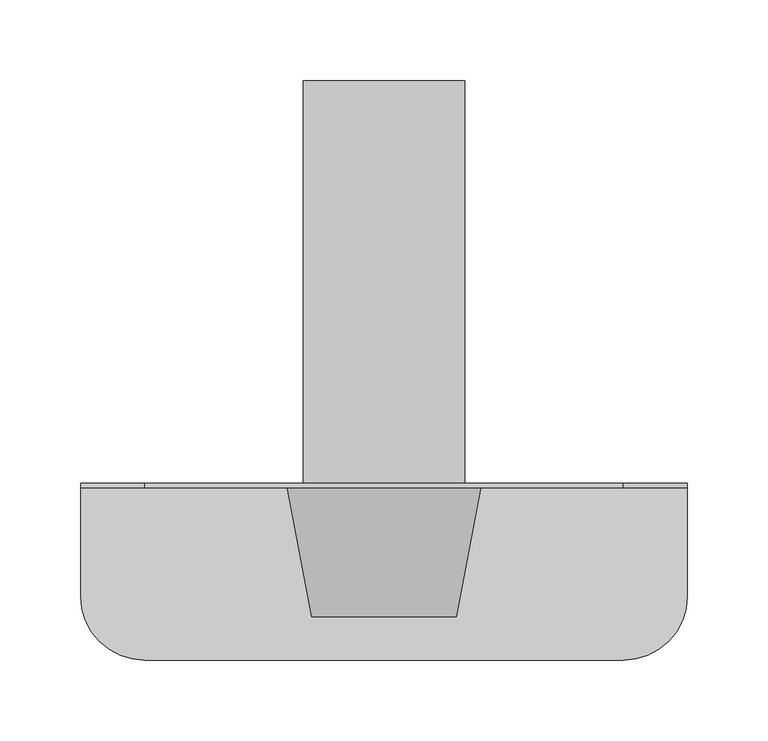
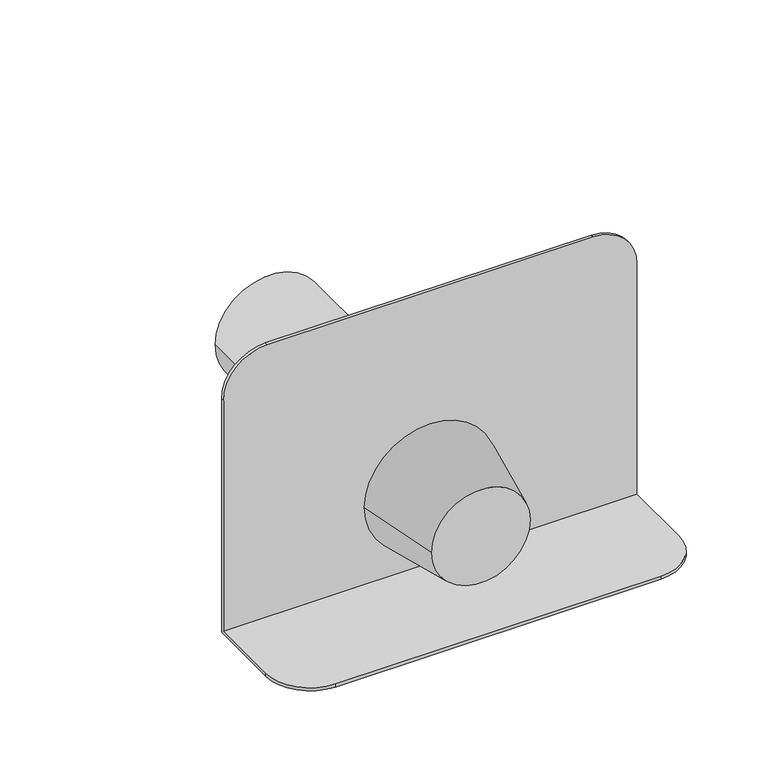
"""IFC4 building model written with IfcOpenShell, lengths in millimetres: proxy geometry, TN_Воронка парапетная ТехноНИКОЛЬ круглая_Тип 1 : Воронка ULTRA парапетная 110 ТехноНИКОЛЬ."""

from ifc_helpers import new_model, si_unit, frame, origin, place, context, project, spatial, polyline, circle_curve, source, transform, mapped, element, save
from ifc_brep_helpers import plane_surface, cylinder_surface, revolved_surface, advanced_brep


def specialty_equipment_830a0a6e(model_context):
    return source(origin(), model_context, "Body", "AdvancedBrep", [
        advanced_brep(
        [(-45.0, -83.0, 77.0), (45.0, -83.0, 77.0), (-60.0, -3.0, 77.0), (60.0, -3.0, 77.0)],
        [
            (0, 1, circle_curve(frame((0.0, -83.0, 77.0), z_axis=(0.0, -1.0, 0.0), x_axis=(-1.0, 0.0, 0.0)), 45.0)),
            (1, 0, circle_curve(frame((0.0, -83.0, 77.0), z_axis=(0.0, -1.0, 0.0), x_axis=(1.0, 0.0, 0.0)), 45.0)),
            (2, 3, circle_curve(frame((0.0, -3.0, 77.0), z_axis=(0.0, 1.0, 0.0), x_axis=(1.0, 0.0, 0.0)), 60.0)),
            (3, 2, circle_curve(frame((0.0, -3.0, 77.0), z_axis=(0.0, 1.0, 0.0), x_axis=(-1.0, 0.0, 0.0)), 60.0)),
            (3, 1),
            (0, 2),
        ],
        [
            plane_surface(frame((0.0, -83.0, 77.0), z_axis=(0.0, -1.0, 0.0), x_axis=(0.0, 0.0, -1.0))),
            plane_surface(frame((0.0, -3.0, 77.0), z_axis=(0.0, 1.0, 0.0), x_axis=(0.0, 0.0, -1.0))),
            revolved_surface(polyline([(-45.0, -83.0, 77.0), (-60.0, -3.0, 77.0)]), (0.0, -323.0, 77.0), (0.0, 1.0, 0.0)),
            revolved_surface(polyline([(45.0, -83.0, 77.0), (60.0, -3.0, 77.0)]), (0.0, -323.0, 77.0), (0.0, 1.0, 0.0)),
        ],
        [
            (0, [[1, 2]]),
            (1, [[3, 4]]),
            (2, [[-4, 5, -1, 6]]),
            (3, [[-3, -6, -2, -5]]),
        ],
    ),
        advanced_brep(
        [(-188.5, -70.0, 3.0), (-148.5, -110.0, 3.0), (148.5, -110.0, 3.0), (188.5, -70.0, 3.0), (188.5, -3.0, 3.0), (-188.5, -3.0, 3.0), (-188.5, 0.0, 0.0), (188.5, 0.0, 0.0), (188.5, -70.0, 0.0), (148.5, -110.0, 0.0), (-148.5, -110.0, 0.0), (-188.5, -70.0, 0.0), (188.5, 0.0, 225.0), (188.5, -3.0, 225.0), (-188.5, 0.0, 225.0), (-148.5, 0.0, 265.0), (148.5, 0.0, 265.0), (-50.0, 0.0, 77.0), (50.0, 0.0, 77.0), (-188.5, -3.0, 225.0), (148.5, -3.0, 265.0), (-148.5, -3.0, 265.0), (-47.0, -3.0, 77.0), (47.0, -3.0, 77.0), (-47.0, 0.0, 77.0), (47.0, 0.0, 77.0), (-50.0, 250.0, 77.0), (50.0, 250.0, 77.0), (-47.0, 250.0, 77.0), (47.0, 250.0, 77.0)],
        [
            (0, 1, circle_curve(frame((-148.5, -70.0, 3.0), z_axis=(0.0, 0.0, 1.0), x_axis=(1.0, 0.0, 0.0)), 40.0)),
            (1, 2),
            (2, 3, circle_curve(frame((148.5, -70.0, 3.0), z_axis=(0.0, 0.0, 1.0), x_axis=(1.0, 0.0, 0.0)), 40.0)),
            (3, 4),
            (4, 5),
            (5, 0),
            (6, 7),
            (7, 8),
            (8, 9, circle_curve(frame((148.5, -70.0, 0.0), z_axis=(0.0, 0.0, -1.0), x_axis=(1.0, 0.0, 0.0)), 40.0)),
            (9, 10),
            (10, 11, circle_curve(frame((-148.5, -70.0, 0.0), z_axis=(0.0, 0.0, -1.0), x_axis=(1.0, 0.0, 0.0)), 40.0)),
            (11, 6),
            (0, 11),
            (10, 1),
            (9, 2),
            (8, 3),
            (7, 12),
            (12, 13),
            (13, 4),
            (6, 14),
            (14, 15, circle_curve(frame((-148.5, 0.0, 225.0), z_axis=(0.0, 1.0, 0.0), x_axis=(1.0, 0.0, 0.0)), 40.0)),
            (15, 16),
            (16, 12, circle_curve(frame((148.5, 0.0, 225.0), z_axis=(0.0, 1.0, 0.0), x_axis=(1.0, 0.0, 0.0)), 40.0)),
            (17, 18, circle_curve(frame((0.0, 0.0, 77.0), z_axis=(0.0, -1.0, 0.0), x_axis=(1.0, 0.0, 0.0)), 50.0)),
            (18, 17, circle_curve(frame((0.0, 0.0, 77.0), z_axis=(0.0, -1.0, 0.0), x_axis=(1.0, 0.0, 0.0)), 50.0)),
            (5, 19),
            (19, 14),
            (13, 20, circle_curve(frame((148.5, -3.0, 225.0), z_axis=(0.0, -1.0, 0.0), x_axis=(1.0, 0.0, 0.0)), 40.0)),
            (20, 21),
            (21, 19, circle_curve(frame((-148.5, -3.0, 225.0), z_axis=(0.0, -1.0, 0.0), x_axis=(1.0, 0.0, 0.0)), 40.0)),
            (22, 23, circle_curve(frame((0.0, -3.0, 77.0), z_axis=(0.0, 1.0, 0.0), x_axis=(1.0, 0.0, 0.0)), 47.0)),
            (23, 22, circle_curve(frame((0.0, -3.0, 77.0), z_axis=(0.0, 1.0, 0.0), x_axis=(1.0, 0.0, 0.0)), 47.0)),
            (16, 20),
            (15, 21),
            (22, 24),
            (24, 25, circle_curve(frame((0.0, 0.0, 77.0), z_axis=(0.0, 1.0, 0.0), x_axis=(1.0, 0.0, 0.0)), 47.0)),
            (25, 23),
            (25, 24, circle_curve(frame((0.0, 0.0, 77.0), z_axis=(0.0, 1.0, 0.0), x_axis=(1.0, 0.0, 0.0)), 47.0)),
            (26, 27, circle_curve(frame((0.0, 250.0, 77.0), z_axis=(0.0, 1.0, 0.0), x_axis=(1.0, 0.0, 0.0)), 50.0)),
            (27, 26, circle_curve(frame((0.0, 250.0, 77.0), z_axis=(0.0, 1.0, 0.0), x_axis=(1.0, 0.0, 0.0)), 50.0)),
            (28, 29, circle_curve(frame((0.0, 250.0, 77.0), z_axis=(0.0, -1.0, 0.0), x_axis=(1.0, 0.0, 0.0)), 47.0)),
            (29, 28, circle_curve(frame((0.0, 250.0, 77.0), z_axis=(0.0, -1.0, 0.0), x_axis=(1.0, 0.0, 0.0)), 47.0)),
            (27, 18),
            (17, 26),
            (29, 25),
            (24, 28),
        ],
        [
            plane_surface(frame((-108.5, -70.0, 3.0), z_axis=(0.0, 0.0, 1.0), x_axis=(0.0, 1.0, 0.0))),
            plane_surface(frame((-108.5, -70.0, 0.0), z_axis=(0.0, 0.0, -1.0), x_axis=(0.0, -1.0, 0.0))),
            cylinder_surface(frame((-148.5, -70.0, 0.0), z_axis=(0.0, 0.0, 1.0), x_axis=(1.0, 0.0, 0.0)), 40.0),
            plane_surface(frame((-148.5, -110.0, 3.0), z_axis=(0.0, -1.0, 0.0), x_axis=(0.0, 0.0, -1.0))),
            cylinder_surface(frame((148.5, -70.0, 0.0), z_axis=(0.0, 0.0, 1.0), x_axis=(1.0, 0.0, 0.0)), 40.0),
            plane_surface(frame((188.5, -70.0, 3.0), z_axis=(1.0, 0.0, 0.0), x_axis=(0.0, 0.0, -1.0))),
            plane_surface(frame((188.5, 0.0, 3.0), z_axis=(0.0, 1.0, 0.0), x_axis=(0.0, 0.0, -1.0))),
            plane_surface(frame((-188.5, 0.0, 3.0), z_axis=(-1.0, 0.0, 0.0), x_axis=(0.0, 0.0, -1.0))),
            plane_surface(frame((-188.5, -3.0, 0.0), z_axis=(0.0, -1.0, 0.0), x_axis=(1.0, 0.0, 0.0))),
            cylinder_surface(frame((148.5, 0.0, 225.0), z_axis=(0.0, -1.0, 0.0), x_axis=(1.0, 0.0, 0.0)), 40.0),
            plane_surface(frame((148.5, -3.0, 265.0), z_axis=(0.0, 0.0, 1.0), x_axis=(0.0, 1.0, 0.0))),
            cylinder_surface(frame((-148.5, 0.0, 225.0), z_axis=(0.0, -1.0, 0.0), x_axis=(1.0, 0.0, 0.0)), 40.0),
            revolved_surface(polyline([(47.0, 0.0, 77.0), (47.0, -3.0, 77.0)]), (0.0, 0.0, 77.0), (0.0, 1.0, 0.0)),
            plane_surface(frame((50.0, 250.0, 77.0), z_axis=(0.0, 1.0, 0.0), x_axis=(0.0, 0.0, -1.0))),
            cylinder_surface(frame((0.0, 250.0, 77.0), z_axis=(0.0, -1.0, 0.0), x_axis=(1.0, 0.0, 0.0)), 50.0),
            revolved_surface(polyline([(47.0, 250.0, 77.0), (47.0, 0.0, 77.0)]), (0.0, 0.0, 77.0), (0.0, 1.0, 0.0)),
        ],
        [
            (0, [[1, 2, 3, 4, 5, 6]]),
            (1, [[7, 8, 9, 10, 11, 12]]),
            (2, [[-1, 13, -11, 14]]),
            (3, [[-2, -14, -10, 15]]),
            (4, [[-3, -15, -9, 16]]),
            (5, [[-16, -8, 17, 18, 19, -4]]),
            (6, [[-7, 20, 21, 22, 23, -17], [24, 25]]),
            (7, [[-13, -6, 26, 27, -20, -12]]),
            (8, [[28, 29, 30, -26, -5, -19], [31, 32]]),
            (9, [[-28, -18, -23, 33]]),
            (10, [[-29, -33, -22, 34]]),
            (11, [[-30, -34, -21, -27]]),
            (12, [[-31, 35, 36, 37]]),
            (12, [[-32, -37, 38, -35]]),
            (13, [[39, 40], [41, 42]]),
            (14, [[-40, 43, -24, 44]]),
            (14, [[-39, -44, -25, -43]]),
            (15, [[-42, 45, -36, 46]]),
            (15, [[-41, -46, -38, -45]]),
        ],
    ),
    ])


if __name__ == "__main__":
    model = new_model("IFC4")
    model_context = context("Model", 3, world=origin())
    ifc_project = project(units=[si_unit("LENGTHUNIT", "METRE", prefix="MILLI")], contexts=[model_context])
    site = spatial("IfcSite", under=ifc_project)
    building = spatial("IfcBuilding", under=site)
    placement = place(None, origin())
    specialty_equipment_shape = specialty_equipment_830a0a6e(model_context)
    element("IfcBuildingElementProxy", 1, Name="TN_Воронка парапетная ТехноНИКОЛЬ круглая_Тип 1 : Воронка ULTRA парапетная 110 ТехноНИКОЛЬ", ObjectType="TN_Воронка парапетная ТехноНИКОЛЬ круглая_Тип 1 : Воронка ULTRA парапетная 110 ТехноНИКОЛЬ", at=placement, inside=building, context=model_context, shape_type="MappedRepresentation", body=[
        mapped(specialty_equipment_shape, transform((0.0, 0.0, 0.0), x_axis=(1.0, 0.0, 0.0), y_axis=(0.0, 1.0, 0.0), z_axis=(0.0, 0.0, 1.0))),
    ])
    save(model, "model.ifc")

# Revit data of these elements
# Type "TN_Воронка парапетная ТехноНИКОЛЬ круглая_Тип 1 : Воронка ULTRA парапетная 110 ТехноНИКОЛЬ"
#   ADSK_Группирование = "Комплектующие и воронки"
#   Description = "Воронка  ULTRA парапетная 110 – воронка является парапетным переливом, которая устанавливается в случаях аварийного сброса воды при засорении основной воронки внутреннего водостока. Воронка имеет круглый диаметр отводящей трубы и изготавливается из полимеров. Пропуская способность 8 л/сек."
#   Manufacturer = "ТехноНИКОЛЬ"
#   URL = "http://nav.tn.ru/catalog/krovlya/vodostochnaya-sistema/parapetnaya-voronka-tekhnonikol/"
#   ADSK_Примечание = ""
#   ADSK_Обозначение = "ТехноНИКОЛЬ"
#   ADSK_Наименование = "Воронка ULTRA парапетная 110 ТехноНИКОЛЬ"
#   ADSK_Марка = ""
#   ADSK_Код изделия = "398253"
#   ADSK_Завод-изготовитель = "ТехноНИКОЛЬ"
#   ADSK_Единица измерения = "шт."
#   ADSK_Группирование = "Комплектующие и воронки"
#   ADSK_URL страницы изделия = "https://shop.tn.ru/voronka-ultra-parapetnaja-110-mm"
#   ADSK_URL документации изделия = "https://nav.tn.ru/upload/iblock/c5b/Tekhlist-7.32-Parapetnaya-voronka_rus.pdf"
#   Ширина фланца = 377 mm
#   Размер фланца по вертикали = 265 mm
#   Длина расчетная [instance default] = 250 mm
#   Длина отвода [instance default] = 250 mm
#   Размер фланца по горизонтали = 110 mm
#   ADSK_Масса = 0.5
#   ADSK_Количество = 1
#   Тип воронки = 1
#   Видимость_Переход [instance default] = no
#   Видимость_Листоуловитель [instance default] = no
#   Материал = TN_ПВХ_Черный
#   Default Elevation = 0
# Element 1 (IfcBuildingElementProxy, "TN_Воронка парапетная ТехноНИКОЛЬ круглая_Тип 1 : Воронка ULTRA парапетная 110 ТехноНИКОЛЬ")
#   Длина отвода = 600 mm
#   Видимость_Листоуловитель = yes
#   Materials on its faces: "TN_ПВХ_Черный"
# Materials
#   "TN_ПВХ_Черный": class "Типовые", colour RGB 48 48 48, transparency 0, Cost = 0
